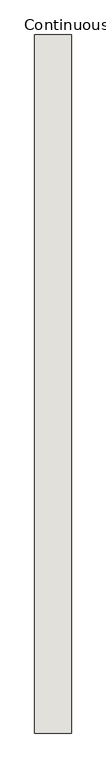
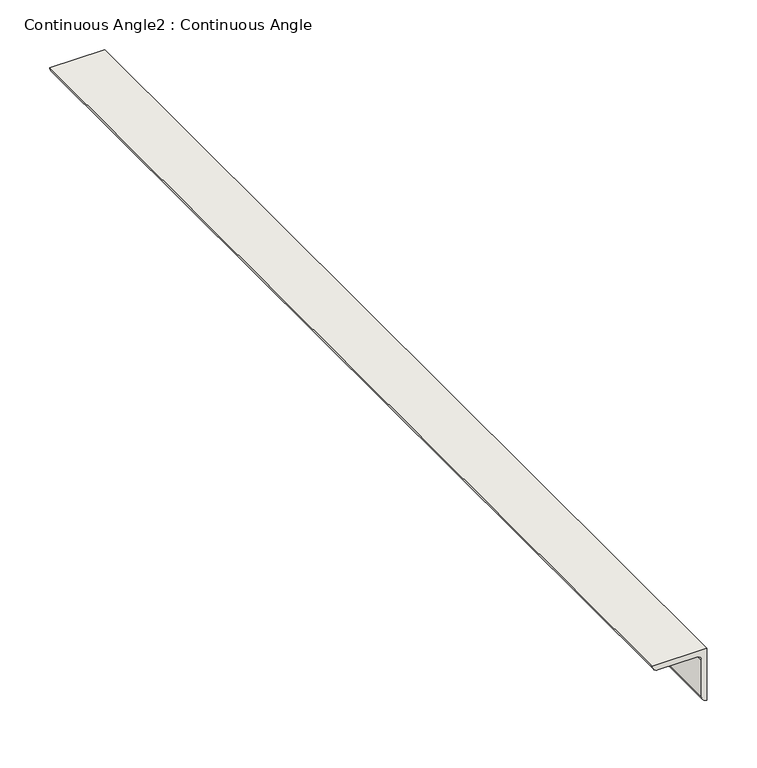
"""IFC4 building model written with IfcOpenShell, lengths in millimetres: wall geometry, Continuous Angle2 : Continuous Angle."""

from ifc_helpers import new_model, si_unit, point, frame, frame_2d, origin, place, context, project, spatial, polyline, circle_curve, trimmed, segment, composite_curve, outline, extrude, source, transform, mapped, element, save


def continuous_angle2_continuous_angle_272cff5c(model_context):
    return source(origin(), model_context, "Body", "SweptSolid", [
        extrude(outline(composite_curve([segment(polyline([(2260.6, 428785.3375), (2260.6, 428721.8375)]), True, "CONTINUOUS"), segment(trimmed(circle_curve(frame_2d((2260.6, 428728.1875)), 6.35), [point((2260.6, 428721.8375))], [point((2254.25, 428728.1875))], False, "CARTESIAN"), True, "CONTINUOUS"), segment(polyline([(2254.25, 428728.1875), (2254.25, 428772.6375)]), True, "CONTINUOUS"), segment(trimmed(circle_curve(frame_2d((2247.9, 428772.6375)), 6.35), [point((2254.25, 428772.6375))], [point((2247.9, 428778.9875))], True, "CARTESIAN"), True, "CONTINUOUS"), segment(polyline([(2247.9, 428778.9875), (2203.45, 428778.9875)]), True, "CONTINUOUS"), segment(trimmed(circle_curve(frame_2d((2203.45, 428785.3375)), 6.35), [point((2203.45, 428778.9875))], [point((2197.1, 428785.3375))], False, "CARTESIAN"), True, "CONTINUOUS"), segment(polyline([(2197.1, 428785.3375), (2260.6, 428785.3375)]), True, "CONTINUOUS")], self_intersect=False)), frame((0.0, 304.8, 0.0), z_axis=(0.0, 1.0, 0.0), x_axis=(0.0, 0.0, 1.0)), (0.0, 0.0, 1.0), 1209.675),
    ])


if __name__ == "__main__":
    model = new_model("IFC4")
    model_context = context("Model", 3, world=origin())
    ifc_project = project(units=[si_unit("LENGTHUNIT", "METRE", prefix="MILLI")], contexts=[model_context])
    site = spatial("IfcSite", under=ifc_project)
    building = spatial("IfcBuilding", under=site)
    placement = place(None, origin())
    continuous_angle2_continuous_angle_shape = continuous_angle2_continuous_angle_272cff5c(model_context)
    element("IfcWall", 1, ObjectType="Continuous Angle2 : Continuous Angle", at=placement, inside=building, context=model_context, shape_type="MappedRepresentation", body=[
        mapped(continuous_angle2_continuous_angle_shape, transform((0.0, 0.0, 0.0), x_axis=(1.0, 0.0, 0.0), y_axis=(0.0, 1.0, 0.0), z_axis=(0.0, 0.0, 1.0))),
    ])
    save(model, "model.ifc")

# Revit data of these elements
# Element 1 (IfcWall, "Continuous Angle2 : Continuous Angle")
#   Materials on its faces: "3\" X 3\" X 8\" L. CLIP ANGLES @ 4'-0\" O.C. MECH. FASTENED TO UNDERSIDE OF STRUCTURE OR SLAB - BOTH SIDES OF WALL"
# Materials
#   "3\" X 3\" X 8\" L. CLIP ANGLES @ 4'-0\" O.C. MECH. FASTENED TO UNDERSIDE OF STRUCTURE OR SLAB - BOTH SIDES OF WALL": class "Unassigned", colour RGB 210 209 208, transparency 0, Keynote = "M05121300.02", Cost = 0
